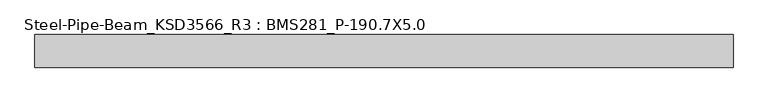
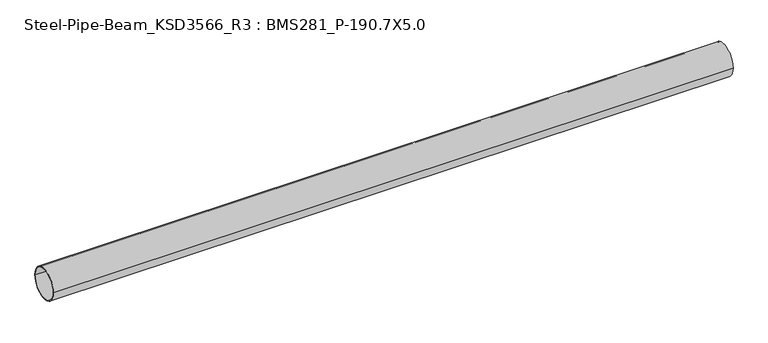
"""IFC4 building model written with IfcOpenShell, lengths in millimetres: member geometry, Steel-Pipe-Beam_KSD3566_R3 : BMS281_P-190.7X5.0."""

from ifc_helpers import new_model, si_unit, point, frame, origin, origin_2d, place, context, project, spatial, circle_curve, trimmed, segment, composite_curve, outline, extrude, source, transform, mapped, element, save


def steel_pipe_beam_ksd3566_r3_bms281_p_190_7x5_0_0fc3a4e3(model_context):
    return source(origin(), model_context, "Body", "SweptSolid", [
        extrude(outline(composite_curve([segment(trimmed(circle_curve(origin_2d(), 95.35), [point((-95.35, 0.0))], [point((95.35, 0.0))], False, "CARTESIAN"), True, "CONTINUOUS"), segment(trimmed(circle_curve(origin_2d(), 95.35), [point((95.35, 0.0))], [point((-95.35, 0.0))], False, "CARTESIAN"), True, "CONTINUOUS")], self_intersect=False), holes=[composite_curve([segment(trimmed(circle_curve(origin_2d(), 90.35), [point((90.35, 0.0))], [point((-90.35, 0.0))], True, "CARTESIAN"), True, "CONTINUOUS"), segment(trimmed(circle_curve(origin_2d(), 90.35), [point((-90.35, 0.0))], [point((90.35, 0.0))], True, "CARTESIAN"), True, "CONTINUOUS")], self_intersect=False)]), frame((-2028.8814264, 0.0, 0.0), z_axis=(1.0, 0.0, 0.0), x_axis=(0.0, 1.0, 0.0)), (0.0, 0.0, 1.0), 4075.0090764),
    ])


if __name__ == "__main__":
    model = new_model("IFC4")
    model_context = context("Model", 3, world=origin())
    ifc_project = project(units=[si_unit("LENGTHUNIT", "METRE", prefix="MILLI")], contexts=[model_context])
    site = spatial("IfcSite", under=ifc_project)
    building = spatial("IfcBuilding", under=site)
    placement = place(None, origin())
    steel_pipe_beam_ksd3566_r3_bms281_p_190_7x5_0_shape = steel_pipe_beam_ksd3566_r3_bms281_p_190_7x5_0_0fc3a4e3(model_context)
    element("IfcMember", 1, ObjectType="Steel-Pipe-Beam_KSD3566_R3 : BMS281_P-190.7X5.0", at=placement, inside=building, context=model_context, shape_type="MappedRepresentation", body=[
        mapped(steel_pipe_beam_ksd3566_r3_bms281_p_190_7x5_0_shape, transform((0.0, 0.0, 0.0), x_axis=(1.0, 0.0, 0.0), y_axis=(0.0, 1.0, 0.0), z_axis=(0.0, 0.0, 1.0))),
    ])
    save(model, "model.ifc")

# Revit data of these elements
# Type "Steel-Pipe-Beam_KSD3566_R3 : BMS281_P-190.7X5.0"
#   Keynote = "P-190.7X5.0"
#   SteelWeight = "Light"
#   t = 0.0050 m
#   Surface Area = 0.599102 m²/m
#   Section Area = 29.1697 cm²
#   Mass per Unit Length = 22.8982 kg/m
#   Length [instance default] = 1.5000 m
#   D = 0.1907 m
#   hec_material4 [instance default] = none
#   hec_material3 [instance default] = none
#   hec_material2 [instance default] = none
#   hec_material1 [instance default] = none
#   Structural Material [instance default] = Steel, 45-345
#   Assembly Code = ""
# Element 1 (IfcMember, "Steel-Pipe-Beam_KSD3566_R3 : BMS281_P-190.7X5.0")
#   Structural Material = none
# Materials
#   "Steel, 45-345": class "Metal", colour RGB 189 187 185, transparency 0, Description = "Steel 345 MPa", Cost = 0
